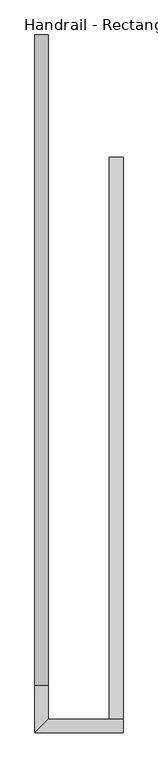
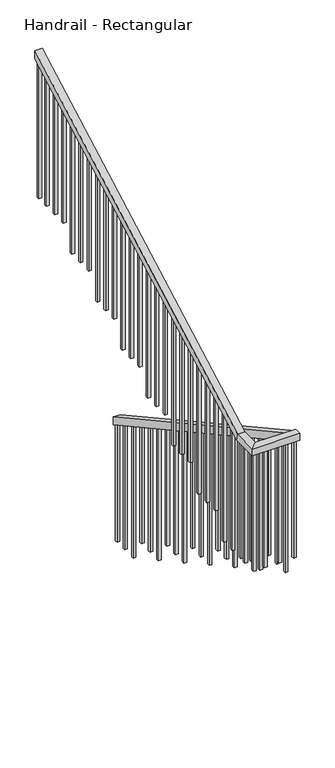
"""IFC4 building model written with IfcOpenShell, lengths in millimetres: railing geometry, Handrail - Rectangular."""

from ifc_helpers import new_model, si_unit, frame, origin, place, context, project, spatial, polyline, outline, extrude, faceted_brep, source, transform, mapped, element, save


def handrail_rectangular_2f1847cf(model_context):
    return source(origin(), model_context, "Body", "SolidModel", [
        faceted_brep([(-74523.6, 12185.65, 17490.1411765), (-74472.8, 12185.65, 17490.1411765), (-74472.8, 12185.65, 17432.1885835), (-74523.6, 12185.65, 17432.1885835), (-74523.6, 10077.45, 18647.5843137), (-74523.6, 10077.45, 18589.6317207), (-74472.8, 10077.45, 18589.6317207), (-74472.8, 10077.45, 18647.5843137)], [[[0, 1, 2, 3]], [[4, 5, 6, 7]], [[1, 0, 4, 7]], [[2, 1, 7, 6]], [[3, 2, 6, 5]], [[0, 3, 5, 4]]]),
        faceted_brep([(-74472.8, 10077.45, 18661.5294118), (-74472.8, 10026.65, 18661.5294118), (-74472.8, 10026.65, 18610.7294118), (-74472.8, 10077.45, 18610.7294118), (-74752.2, 10077.45, 18661.5294118), (-74803.0, 10026.65, 18661.5294118), (-74803.0, 10026.65, 18610.7294118), (-74752.2, 10077.45, 18610.7294118), (-74752.2, 10204.45, 18661.5294118), (-74803.0, 10204.45, 18661.5294118), (-74803.0, 10217.4779373, 18610.7294118), (-74752.2, 10217.4779373, 18610.7294118), (-74752.2, 12642.85, 20000.2588235), (-74752.2, 12642.85, 19942.3062305), (-74803.0, 12642.85, 19942.3062305), (-74803.0, 12642.85, 20000.2588235)], [[[0, 1, 2, 3]], [[1, 0, 4, 5]], [[2, 1, 5, 6]], [[3, 2, 6, 7]], [[0, 3, 7, 4]], [[5, 4, 8, 9]], [[6, 5, 9, 10]], [[7, 6, 10, 11]], [[4, 7, 11, 8]], [[12, 13, 14, 15]], [[9, 8, 12, 15]], [[10, 9, 15, 14]], [[11, 10, 14, 13]], [[8, 11, 13, 12]]]),
        extrude(outline(polyline([(12531.725, 19881.2964266), (12550.775, 19891.7552501), (12550.775, 18918.5176471), (12531.725, 18918.5176471), (12531.725, 19881.2964266)])), frame((-74787.125, 0.0, 0.0), z_axis=(1.0, 0.0, 0.0), x_axis=(0.0, 1.0, 0.0)), (0.0, 0.0, 1.0), 19.05),
        extrude(outline(polyline([(12430.125, 19825.5160344), (12449.175, 19835.974858), (12449.175, 18918.5176471), (12430.125, 18918.5176471), (12430.125, 19825.5160344)])), frame((-74787.125, 0.0, 0.0), z_axis=(1.0, 0.0, 0.0), x_axis=(0.0, 1.0, 0.0)), (0.0, 0.0, 1.0), 19.05),
        extrude(outline(polyline([(12328.525, 19769.7356423), (12347.575, 19780.1944658), (12347.575, 18918.5176471), (12328.525, 18918.5176471), (12328.525, 19769.7356423)])), frame((-74787.125, 0.0, 0.0), z_axis=(1.0, 0.0, 0.0), x_axis=(0.0, 1.0, 0.0)), (0.0, 0.0, 1.0), 19.05),
        extrude(outline(polyline([(12226.925, 19713.9552501), (12245.975, 19724.4140737), (12245.975, 18751.1764706), (12226.925, 18751.1764706), (12226.925, 19713.9552501)])), frame((-74787.125, 0.0, 0.0), z_axis=(1.0, 0.0, 0.0), x_axis=(0.0, 1.0, 0.0)), (0.0, 0.0, 1.0), 19.05),
        extrude(outline(polyline([(12125.325, 19658.174858), (12144.375, 19668.6336815), (12144.375, 18751.1764706), (12125.325, 18751.1764706), (12125.325, 19658.174858)])), frame((-74787.125, 0.0, 0.0), z_axis=(1.0, 0.0, 0.0), x_axis=(0.0, 1.0, 0.0)), (0.0, 0.0, 1.0), 19.05),
        extrude(outline(polyline([(12023.725, 19602.3944658), (12042.775, 19612.8532893), (12042.775, 18751.1764706), (12023.725, 18751.1764706), (12023.725, 19602.3944658)])), frame((-74787.125, 0.0, 0.0), z_axis=(1.0, 0.0, 0.0), x_axis=(0.0, 1.0, 0.0)), (0.0, 0.0, 1.0), 19.05),
        extrude(outline(polyline([(11922.125, 19546.6140737), (11941.175, 19557.0728972), (11941.175, 18583.8352941), (11922.125, 18583.8352941), (11922.125, 19546.6140737)])), frame((-74787.125, 0.0, 0.0), z_axis=(1.0, 0.0, 0.0), x_axis=(0.0, 1.0, 0.0)), (0.0, 0.0, 1.0), 19.05),
        extrude(outline(polyline([(11820.525, 19490.8336815), (11839.575, 19501.292505), (11839.575, 18583.8352941), (11820.525, 18583.8352941), (11820.525, 19490.8336815)])), frame((-74787.125, 0.0, 0.0), z_axis=(1.0, 0.0, 0.0), x_axis=(0.0, 1.0, 0.0)), (0.0, 0.0, 1.0), 19.05),
        extrude(outline(polyline([(11718.925, 19435.0532893), (11737.975, 19445.5121129), (11737.975, 18583.8352941), (11718.925, 18583.8352941), (11718.925, 19435.0532893)])), frame((-74787.125, 0.0, 0.0), z_axis=(1.0, 0.0, 0.0), x_axis=(0.0, 1.0, 0.0)), (0.0, 0.0, 1.0), 19.05),
        extrude(outline(polyline([(11617.325, 19379.2728972), (11636.375, 19389.7317207), (11636.375, 18416.4941176), (11617.325, 18416.4941176), (11617.325, 19379.2728972)])), frame((-74787.125, 0.0, 0.0), z_axis=(1.0, 0.0, 0.0), x_axis=(0.0, 1.0, 0.0)), (0.0, 0.0, 1.0), 19.05),
        extrude(outline(polyline([(11515.725, 19323.492505), (11534.775, 19333.9513286), (11534.775, 18416.4941176), (11515.725, 18416.4941176), (11515.725, 19323.492505)])), frame((-74787.125, 0.0, 0.0), z_axis=(1.0, 0.0, 0.0), x_axis=(0.0, 1.0, 0.0)), (0.0, 0.0, 1.0), 19.05),
        extrude(outline(polyline([(11414.125, 19267.7121129), (11433.175, 19278.1709364), (11433.175, 18416.4941176), (11414.125, 18416.4941176), (11414.125, 19267.7121129)])), frame((-74787.125, 0.0, 0.0), z_axis=(1.0, 0.0, 0.0), x_axis=(0.0, 1.0, 0.0)), (0.0, 0.0, 1.0), 19.05),
        extrude(outline(polyline([(11312.525, 19211.9317207), (11331.575, 19222.3905442), (11331.575, 18249.1529412), (11312.525, 18249.1529412), (11312.525, 19211.9317207)])), frame((-74787.125, 0.0, 0.0), z_axis=(1.0, 0.0, 0.0), x_axis=(0.0, 1.0, 0.0)), (0.0, 0.0, 1.0), 19.05),
        extrude(outline(polyline([(11210.925, 19156.1513286), (11229.975, 19166.6101521), (11229.975, 18249.1529412), (11210.925, 18249.1529412), (11210.925, 19156.1513286)])), frame((-74787.125, 0.0, 0.0), z_axis=(1.0, 0.0, 0.0), x_axis=(0.0, 1.0, 0.0)), (0.0, 0.0, 1.0), 19.05),
        extrude(outline(polyline([(11109.325, 19100.3709364), (11128.375, 19110.8297599), (11128.375, 18249.1529412), (11109.325, 18249.1529412), (11109.325, 19100.3709364)])), frame((-74787.125, 0.0, 0.0), z_axis=(1.0, 0.0, 0.0), x_axis=(0.0, 1.0, 0.0)), (0.0, 0.0, 1.0), 19.05),
        extrude(outline(polyline([(11007.725, 19044.5905442), (11026.775, 19055.0493678), (11026.775, 18081.8117647), (11007.725, 18081.8117647), (11007.725, 19044.5905442)])), frame((-74787.125, 0.0, 0.0), z_axis=(1.0, 0.0, 0.0), x_axis=(0.0, 1.0, 0.0)), (0.0, 0.0, 1.0), 19.05),
        extrude(outline(polyline([(10906.125, 18988.8101521), (10925.175, 18999.2689756), (10925.175, 18081.8117647), (10906.125, 18081.8117647), (10906.125, 18988.8101521)])), frame((-74787.125, 0.0, 0.0), z_axis=(1.0, 0.0, 0.0), x_axis=(0.0, 1.0, 0.0)), (0.0, 0.0, 1.0), 19.05),
        extrude(outline(polyline([(10804.525, 18933.0297599), (10823.575, 18943.4885835), (10823.575, 18081.8117647), (10804.525, 18081.8117647), (10804.525, 18933.0297599)])), frame((-74787.125, 0.0, 0.0), z_axis=(1.0, 0.0, 0.0), x_axis=(0.0, 1.0, 0.0)), (0.0, 0.0, 1.0), 19.05),
        extrude(outline(polyline([(10702.925, 18877.2493678), (10721.975, 18887.7081913), (10721.975, 17914.4705882), (10702.925, 17914.4705882), (10702.925, 18877.2493678)])), frame((-74787.125, 0.0, 0.0), z_axis=(1.0, 0.0, 0.0), x_axis=(0.0, 1.0, 0.0)), (0.0, 0.0, 1.0), 19.05),
        extrude(outline(polyline([(10601.325, 18821.4689756), (10620.375, 18831.9277991), (10620.375, 17914.4705882), (10601.325, 17914.4705882), (10601.325, 18821.4689756)])), frame((-74787.125, 0.0, 0.0), z_axis=(1.0, 0.0, 0.0), x_axis=(0.0, 1.0, 0.0)), (0.0, 0.0, 1.0), 19.05),
        extrude(outline(polyline([(10499.725, 18765.6885835), (10518.775, 18776.147407), (10518.775, 17914.4705882), (10499.725, 17914.4705882), (10499.725, 18765.6885835)])), frame((-74787.125, 0.0, 0.0), z_axis=(1.0, 0.0, 0.0), x_axis=(0.0, 1.0, 0.0)), (0.0, 0.0, 1.0), 19.05),
        extrude(outline(polyline([(10398.125, 18709.9081913), (10417.175, 18720.3670148), (10417.175, 17747.1294118), (10398.125, 17747.1294118), (10398.125, 18709.9081913)])), frame((-74787.125, 0.0, 0.0), z_axis=(1.0, 0.0, 0.0), x_axis=(0.0, 1.0, 0.0)), (0.0, 0.0, 1.0), 19.05),
        extrude(outline(polyline([(10296.525, 18654.1277991), (10315.575, 18664.5866227), (10315.575, 17747.1294118), (10296.525, 17747.1294118), (10296.525, 18654.1277991)])), frame((-74787.125, 0.0, 0.0), z_axis=(1.0, 0.0, 0.0), x_axis=(0.0, 1.0, 0.0)), (0.0, 0.0, 1.0), 19.05),
        extrude(outline(polyline([(-74768.075, 10144.125), (-74787.125, 10144.125), (-74787.125, 10163.175), (-74768.075, 10163.175), (-74768.075, 10144.125)])), frame((0.0, 0.0, 17747.1294118), z_axis=(0.0, 0.0, 1.0), x_axis=(1.0, 0.0, 0.0)), (0.0, 0.0, 1.0), 863.6),
        extrude(outline(polyline([(-74691.875, 10061.575), (-74691.875, 10042.525), (-74710.925, 10042.525), (-74710.925, 10061.575), (-74691.875, 10061.575)])), frame((0.0, 0.0, 17747.1294118), z_axis=(0.0, 0.0, 1.0), x_axis=(1.0, 0.0, 0.0)), (0.0, 0.0, 1.0), 863.6),
        extrude(outline(polyline([(-74590.275, 10061.575), (-74590.275, 10042.525), (-74609.325, 10042.525), (-74609.325, 10061.575), (-74590.275, 10061.575)])), frame((0.0, 0.0, 17747.1294118), z_axis=(0.0, 0.0, 1.0), x_axis=(1.0, 0.0, 0.0)), (0.0, 0.0, 1.0), 863.6),
        extrude(outline(polyline([(10144.125, 18553.0258384), (10163.175, 18542.5670148), (10163.175, 17579.7882353), (10144.125, 17579.7882353), (10144.125, 18553.0258384)])), frame((-74507.725, 0.0, 0.0), z_axis=(1.0, 0.0, 0.0), x_axis=(0.0, 1.0, 0.0)), (0.0, 0.0, 1.0), 19.05),
        extrude(outline(polyline([(10245.725, 18497.2454462), (10264.775, 18486.7866227), (10264.775, 17579.7882353), (10245.725, 17579.7882353), (10245.725, 18497.2454462)])), frame((-74507.725, 0.0, 0.0), z_axis=(1.0, 0.0, 0.0), x_axis=(0.0, 1.0, 0.0)), (0.0, 0.0, 1.0), 19.05),
        extrude(outline(polyline([(10347.325, 18441.465054), (10366.375, 18431.0062305), (10366.375, 17579.7882353), (10347.325, 17579.7882353), (10347.325, 18441.465054)])), frame((-74507.725, 0.0, 0.0), z_axis=(1.0, 0.0, 0.0), x_axis=(0.0, 1.0, 0.0)), (0.0, 0.0, 1.0), 19.05),
        extrude(outline(polyline([(10448.925, 18385.6846619), (10467.975, 18375.2258384), (10467.975, 17412.4470588), (10448.925, 17412.4470588), (10448.925, 18385.6846619)])), frame((-74507.725, 0.0, 0.0), z_axis=(1.0, 0.0, 0.0), x_axis=(0.0, 1.0, 0.0)), (0.0, 0.0, 1.0), 19.05),
        extrude(outline(polyline([(10550.525, 18329.9042697), (10569.575, 18319.4454462), (10569.575, 17412.4470588), (10550.525, 17412.4470588), (10550.525, 18329.9042697)])), frame((-74507.725, 0.0, 0.0), z_axis=(1.0, 0.0, 0.0), x_axis=(0.0, 1.0, 0.0)), (0.0, 0.0, 1.0), 19.05),
        extrude(outline(polyline([(10652.125, 18274.1238776), (10671.175, 18263.665054), (10671.175, 17412.4470588), (10652.125, 17412.4470588), (10652.125, 18274.1238776)])), frame((-74507.725, 0.0, 0.0), z_axis=(1.0, 0.0, 0.0), x_axis=(0.0, 1.0, 0.0)), (0.0, 0.0, 1.0), 19.05),
        extrude(outline(polyline([(10753.725, 18218.3434854), (10772.775, 18207.8846619), (10772.775, 17245.1058824), (10753.725, 17245.1058824), (10753.725, 18218.3434854)])), frame((-74507.725, 0.0, 0.0), z_axis=(1.0, 0.0, 0.0), x_axis=(0.0, 1.0, 0.0)), (0.0, 0.0, 1.0), 19.05),
        extrude(outline(polyline([(10855.325, 18162.5630933), (10874.375, 18152.1042697), (10874.375, 17245.1058824), (10855.325, 17245.1058824), (10855.325, 18162.5630933)])), frame((-74507.725, 0.0, 0.0), z_axis=(1.0, 0.0, 0.0), x_axis=(0.0, 1.0, 0.0)), (0.0, 0.0, 1.0), 19.05),
        extrude(outline(polyline([(10956.925, 18106.7827011), (10975.975, 18096.3238776), (10975.975, 17245.1058824), (10956.925, 17245.1058824), (10956.925, 18106.7827011)])), frame((-74507.725, 0.0, 0.0), z_axis=(1.0, 0.0, 0.0), x_axis=(0.0, 1.0, 0.0)), (0.0, 0.0, 1.0), 19.05),
        extrude(outline(polyline([(11058.525, 18051.0023089), (11077.575, 18040.5434854), (11077.575, 17077.7647059), (11058.525, 17077.7647059), (11058.525, 18051.0023089)])), frame((-74507.725, 0.0, 0.0), z_axis=(1.0, 0.0, 0.0), x_axis=(0.0, 1.0, 0.0)), (0.0, 0.0, 1.0), 19.05),
        extrude(outline(polyline([(11160.125, 17995.2219168), (11179.175, 17984.7630933), (11179.175, 17077.7647059), (11160.125, 17077.7647059), (11160.125, 17995.2219168)])), frame((-74507.725, 0.0, 0.0), z_axis=(1.0, 0.0, 0.0), x_axis=(0.0, 1.0, 0.0)), (0.0, 0.0, 1.0), 19.05),
        extrude(outline(polyline([(11261.725, 17939.4415246), (11280.775, 17928.9827011), (11280.775, 17077.7647059), (11261.725, 17077.7647059), (11261.725, 17939.4415246)])), frame((-74507.725, 0.0, 0.0), z_axis=(1.0, 0.0, 0.0), x_axis=(0.0, 1.0, 0.0)), (0.0, 0.0, 1.0), 19.05),
        extrude(outline(polyline([(11363.325, 17883.6611325), (11382.375, 17873.2023089), (11382.375, 16910.4235294), (11363.325, 16910.4235294), (11363.325, 17883.6611325)])), frame((-74507.725, 0.0, 0.0), z_axis=(1.0, 0.0, 0.0), x_axis=(0.0, 1.0, 0.0)), (0.0, 0.0, 1.0), 19.05),
        extrude(outline(polyline([(11464.925, 17827.8807403), (11483.975, 17817.4219168), (11483.975, 16910.4235294), (11464.925, 16910.4235294), (11464.925, 17827.8807403)])), frame((-74507.725, 0.0, 0.0), z_axis=(1.0, 0.0, 0.0), x_axis=(0.0, 1.0, 0.0)), (0.0, 0.0, 1.0), 19.05),
        extrude(outline(polyline([(11566.525, 17772.1003482), (11585.575, 17761.6415246), (11585.575, 16910.4235294), (11566.525, 16910.4235294), (11566.525, 17772.1003482)])), frame((-74507.725, 0.0, 0.0), z_axis=(1.0, 0.0, 0.0), x_axis=(0.0, 1.0, 0.0)), (0.0, 0.0, 1.0), 19.05),
        extrude(outline(polyline([(11668.125, 17716.319956), (11687.175, 17705.8611325), (11687.175, 16743.0823529), (11668.125, 16743.0823529), (11668.125, 17716.319956)])), frame((-74507.725, 0.0, 0.0), z_axis=(1.0, 0.0, 0.0), x_axis=(0.0, 1.0, 0.0)), (0.0, 0.0, 1.0), 19.05),
        extrude(outline(polyline([(11769.725, 17660.5395638), (11788.775, 17650.0807403), (11788.775, 16743.0823529), (11769.725, 16743.0823529), (11769.725, 17660.5395638)])), frame((-74507.725, 0.0, 0.0), z_axis=(1.0, 0.0, 0.0), x_axis=(0.0, 1.0, 0.0)), (0.0, 0.0, 1.0), 19.05),
        extrude(outline(polyline([(11871.325, 17604.7591717), (11890.375, 17594.3003482), (11890.375, 16743.0823529), (11871.325, 16743.0823529), (11871.325, 17604.7591717)])), frame((-74507.725, 0.0, 0.0), z_axis=(1.0, 0.0, 0.0), x_axis=(0.0, 1.0, 0.0)), (0.0, 0.0, 1.0), 19.05),
        extrude(outline(polyline([(11972.925, 17548.9787795), (11991.975, 17538.519956), (11991.975, 16575.7411765), (11972.925, 16575.7411765), (11972.925, 17548.9787795)])), frame((-74507.725, 0.0, 0.0), z_axis=(1.0, 0.0, 0.0), x_axis=(0.0, 1.0, 0.0)), (0.0, 0.0, 1.0), 19.05),
        extrude(outline(polyline([(12074.525, 17493.1983874), (12093.575, 17482.7395638), (12093.575, 16575.7411765), (12074.525, 16575.7411765), (12074.525, 17493.1983874)])), frame((-74507.725, 0.0, 0.0), z_axis=(1.0, 0.0, 0.0), x_axis=(0.0, 1.0, 0.0)), (0.0, 0.0, 1.0), 19.05),
        extrude(outline(polyline([(-74768.075, 10194.925), (-74787.125, 10194.925), (-74787.125, 10213.975), (-74768.075, 10213.975), (-74768.075, 10194.925)])), frame((0.0, 0.0, 17747.1294118), z_axis=(0.0, 0.0, 1.0), x_axis=(1.0, 0.0, 0.0)), (0.0, 0.0, 1.0), 863.6),
        extrude(outline(polyline([(-74768.075, 10061.575), (-74768.075, 10042.525), (-74787.125, 10042.525), (-74787.125, 10061.575), (-74768.075, 10061.575)])), frame((0.0, 0.0, 17747.1294118), z_axis=(0.0, 0.0, 1.0), x_axis=(1.0, 0.0, 0.0)), (0.0, 0.0, 1.0), 863.6),
        extrude(outline(polyline([(10042.525, 18608.8062305), (10061.575, 18598.347407), (10061.575, 17747.1294118), (10042.525, 17747.1294118), (10042.525, 18608.8062305)])), frame((-74507.725, 0.0, 0.0), z_axis=(1.0, 0.0, 0.0), x_axis=(0.0, 1.0, 0.0)), (0.0, 0.0, 1.0), 19.05),
        extrude(outline(polyline([(12623.8, 19931.847407), (12642.85, 19942.3062305), (12642.85, 18918.5176471), (12623.8, 18918.5176471), (12623.8, 19931.847407)])), frame((-74787.125, 0.0, 0.0), z_axis=(1.0, 0.0, 0.0), x_axis=(0.0, 1.0, 0.0)), (0.0, 0.0, 1.0), 19.05),
        extrude(outline(polyline([(12166.6, 17442.647407), (12185.65, 17432.1885835), (12185.65, 16575.7411765), (12166.6, 16575.7411765), (12166.6, 17442.647407)])), frame((-74507.725, 0.0, 0.0), z_axis=(1.0, 0.0, 0.0), x_axis=(0.0, 1.0, 0.0)), (0.0, 0.0, 1.0), 19.05),
    ])


if __name__ == "__main__":
    model = new_model("IFC4")
    model_context = context("Model", 3, world=origin())
    ifc_project = project(units=[si_unit("LENGTHUNIT", "METRE", prefix="MILLI")], contexts=[model_context])
    site = spatial("IfcSite", under=ifc_project)
    building = spatial("IfcBuilding", under=site)
    placement = place(None, origin())
    handrail_rectangular_shape = handrail_rectangular_2f1847cf(model_context)
    element("IfcRailing", 1, ObjectType="Handrail - Rectangular", at=placement, inside=building, context=model_context, shape_type="MappedRepresentation", body=[
        mapped(handrail_rectangular_shape, transform((0.0, 0.0, 0.0), x_axis=(1.0, 0.0, 0.0), y_axis=(0.0, 1.0, 0.0), z_axis=(0.0, 0.0, 1.0))),
    ])
    save(model, "model.ifc")
